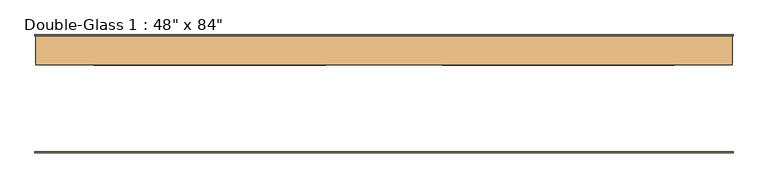
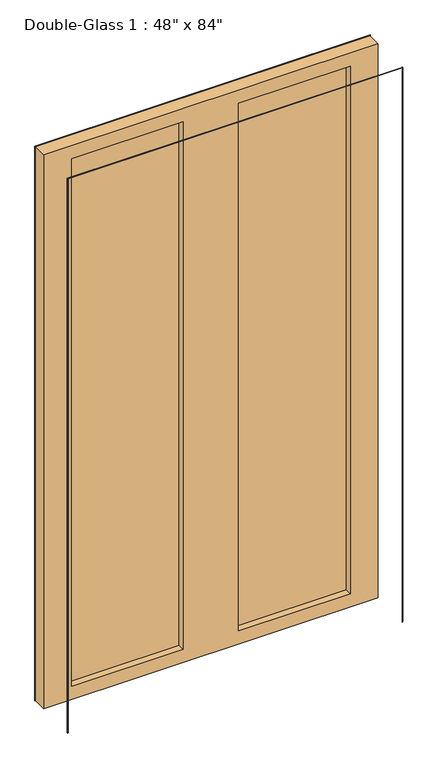
"""IFC4 building model written with IfcOpenShell, lengths in millimetres: door geometry."""

from ifc_helpers import new_model, si_unit, frame, origin, place, context, project, spatial, polyline, outline, extrude, source, transform, mapped, element, save


def door_f7b73743(model_context):
    return source(origin(), model_context, "Body", "SweptSolid", [
        extrude(outline(polyline([(0.0, 611.1875), (2135.1875, 611.1875), (2135.1875, -611.1875), (0.0, -611.1875), (0.0, -609.6), (2133.6, -609.6), (2133.6, 609.6), (0.0, 609.6), (0.0, 611.1875)])), frame((0.0, -100.80625, 0.0), z_axis=(0.0, 1.0, 0.0), x_axis=(0.0, 0.0, 1.0)), (0.0, 0.0, 1.0), 1.5875),
        extrude(outline(polyline([(2133.6, 609.6), (0.0, 609.6), (0.0, 611.1875), (2135.1875, 611.1875), (2135.1875, -611.1875), (0.0, -611.1875), (0.0, -609.6), (2133.6, -609.6), (2133.6, 609.6)])), frame((0.0, 103.98125, 0.0), z_axis=(0.0, 1.0, 0.0), x_axis=(0.0, 0.0, 1.0)), (0.0, 0.0, 1.0), 1.5875),
        extrude(outline(polyline([(508.0, 78.58125), (101.6, 78.58125), (101.6, 85.725), (508.0, 85.725), (508.0, 78.58125)])), frame((0.0, 0.0, 50.8), z_axis=(0.0, 0.0, 1.0), x_axis=(1.0, 0.0, 0.0)), (0.0, 0.0, 1.0), 2032.0),
        extrude(outline(polyline([(-101.6, 78.58125), (-508.0, 78.58125), (-508.0, 85.725), (-101.6, 85.725), (-101.6, 78.58125)])), frame((0.0, 0.0, 50.8), z_axis=(0.0, 0.0, 1.0), x_axis=(1.0, 0.0, 0.0)), (0.0, 0.0, 1.0), 2032.0),
        extrude(outline(polyline([(2133.6, 609.6), (2133.6, -609.6), (0.0, -609.6), (0.0, 609.6), (2133.6, 609.6)]), holes=[polyline([(2082.8, -101.6), (50.8, -101.6), (50.8, -508.0), (2082.8, -508.0), (2082.8, -101.6)]), polyline([(2082.8, 508.0), (50.8, 508.0), (50.8, 101.6), (2082.8, 101.6), (2082.8, 508.0)])]), frame((0.0, 53.18125, 0.0), z_axis=(0.0, 1.0, 0.0), x_axis=(0.0, 0.0, 1.0)), (0.0, 0.0, 1.0), 50.8),
    ])


if __name__ == "__main__":
    model = new_model("IFC4")
    model_context = context("Model", 3, world=origin())
    ifc_project = project(units=[si_unit("LENGTHUNIT", "METRE", prefix="MILLI")], contexts=[model_context])
    site = spatial("IfcSite", under=ifc_project)
    building = spatial("IfcBuilding", under=site)
    placement = place(None, origin())
    door_shape = door_f7b73743(model_context)
    element("IfcDoor", 1, ObjectType="Double-Glass 1 : 48\" x 84\"", at=placement, inside=building, context=model_context, shape_type="MappedRepresentation", body=[
        mapped(door_shape, transform((0.0, 0.0, 0.0), x_axis=(1.0, 0.0, 0.0), y_axis=(0.0, 1.0, 0.0), z_axis=(0.0, 0.0, 1.0))),
    ])
    save(model, "model.ifc")

# Revit data of these elements
# Type "Double-Glass 1 : 48\" x 84\""
#   Type Mark = "21"
#   Assembly Code = "C1020"
#   Thickness = 0' - 2"
#   Height = 7' - 0"
#   Rail Width - Base = 0' - 2"
#   Rail Width - Top = 0' - 2"
#   Stile Width - Hinge = 0' - 2"
#   Stile Width - Latch = 0' - 2"
#   Trim Projection = 0' - 0 1/16"
#   Trim Width = 0' - 0 1/16"
#   Width = 4' - 0"
#   Door Material = Door - Panel
#   Frame Material = Door - Frame
#   Function = (empty or 0)
#   Wall Closure = (empty or 0)
# Element 1 (IfcDoor, "Double-Glass 1 : 48\" x 84\"")
#   Materials on its faces: "Door - Frame", "Door - Panel", "Glass"
# Materials
#   "Door - Panel": class "Wood", colour RGB 210 159 95, transparency 0
#   "Door - Frame": class "Miscellaneous", colour RGB 118 70 51, transparency 0
#   "Glass": class "Glass", colour RGB 0 128 192, transparency 0.75
